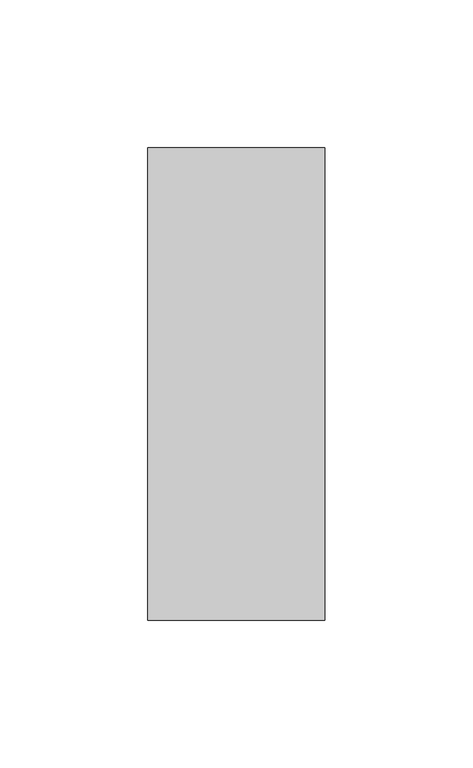
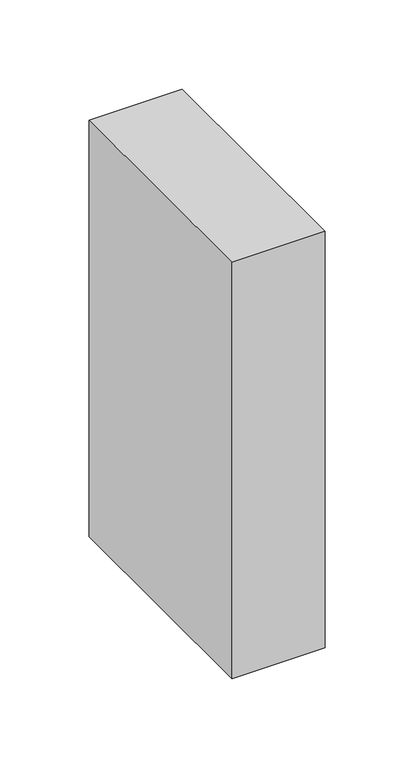
"""IFC4 building model written with IfcOpenShell, lengths in millimetres: column geometry, Madeira de lei-Coluna : Pontalete 6X16cm."""

import ifcopenshell
import ifcopenshell.guid

model = None  # the IFC model being written
_history = None  # IfcOwnerHistory: only IFC2X3 demands one
_inside = {}  # id of a spatial element -> (the spatial element, [elements in it])
_under = {}  # id of a project, library or spatial element -> (it, [spatial elements below it])
_declared = {}  # id of a project -> (the project, [libraries it declares])
_typed = {}  # id of a type object -> (the type object, [elements of that type])
_made_of = {}  # id of a material, layer set ... -> (it, [elements and type objects made of it])


def new_model(schema):
    """Start an empty IFC model of exactly this schema.

    Asked for "IFC4X3", IfcOpenShell would pick the latest addendum, in which some entities
    have other attributes; the version numbers below select the first issue.
    IFC2X3 requires an IfcOwnerHistory on every rooted entity: one is made here for all.
    """
    global model, _history
    if schema == "IFC4X3":
        model = ifcopenshell.file(schema_version=(4, 3, 0, 0))
    else:
        model = ifcopenshell.file(schema=schema)
    _inside.clear()
    _under.clear()
    _declared.clear()
    _typed.clear()
    _made_of.clear()
    _history = None
    if model.schema == "IFC2X3":
        org = make("IfcOrganization", Name="unknown")
        user = make(
            "IfcPersonAndOrganization",
            ThePerson=make("IfcPerson", FamilyName="unknown"),
            TheOrganization=org,
        )
        app = make(
            "IfcApplication",
            ApplicationDeveloper=org,
            Version="unknown",
            ApplicationFullName="unknown",
            ApplicationIdentifier="unknown",
        )
        _history = make(
            "IfcOwnerHistory",
            OwningUser=user,
            OwningApplication=app,
            ChangeAction="ADDED",
            CreationDate=0,
        )
    return model


def make(cls, **values):
    """One entity of the class cls with the attributes given. An attribute that is None is left unset."""
    return model.create_entity(
        cls, **{name: value for name, value in values.items() if value is not None}
    )


def rooted(cls, **values):
    """An entity with a GlobalId (a new one), such as an element, a storey or a relation."""
    return make(cls, GlobalId=ifcopenshell.guid.new(), OwnerHistory=_history, **values)


def si_unit(unit_type, name, prefix=None):
    """IfcSIUnit, for example si_unit("LENGTHUNIT", "METRE", prefix="MILLI")."""
    return make("IfcSIUnit", UnitType=unit_type, Prefix=prefix, Name=name)


def assignment(units):
    """IfcUnitAssignment: the units of a project."""
    return None if units is None else make("IfcUnitAssignment", Units=units)


def point(xyz):
    """IfcCartesianPoint."""
    return None if xyz is None else make("IfcCartesianPoint", Coordinates=xyz)


def direction(xyz):
    """IfcDirection."""
    return None if xyz is None else make("IfcDirection", DirectionRatios=xyz)


def frame(location, z_axis=None, x_axis=None):
    """IfcAxis2Placement3D, a coordinate frame: its origin and axes. An axis left out is left unset."""
    return make(
        "IfcAxis2Placement3D",
        Location=point(location),
        Axis=direction(z_axis),
        RefDirection=direction(x_axis),
    )


def origin():
    """The frame at (0, 0, 0) with its axes left unset."""
    return frame((0.0, 0.0, 0.0))


def place(relative_to, where):
    """IfcLocalPlacement: puts the frame where relative to a parent placement (None: the world)."""
    return make(
        "IfcLocalPlacement", PlacementRelTo=relative_to, RelativePlacement=where
    )


def context(
    kind, dimensions, precision=None, world=None, true_north=None, identifier=None
):
    """IfcGeometricRepresentationContext, for example the 3D "Model" context."""
    return make(
        "IfcGeometricRepresentationContext",
        ContextIdentifier=identifier,
        ContextType=kind,
        CoordinateSpaceDimension=dimensions,
        Precision=precision,
        WorldCoordinateSystem=world,
        TrueNorth=true_north,
    )


def project(units=None, contexts=None):
    """IfcProject with its units and contexts."""
    return rooted(
        "IfcProject",
        Name="project",
        RepresentationContexts=contexts,
        UnitsInContext=assignment(units),
    )


def spatial(cls, under=None, at=None, **own):
    """A site, building, storey or space (cls), placed at a placement, below another one or the project."""
    s = rooted(cls, ObjectPlacement=at, **own)
    if under is not None:
        _under.setdefault(under.id(), (under, []))[1].append(s)
    return s


def polyline(points):
    """IfcPolyline through the points."""
    return make("IfcPolyline", Points=[point(p) for p in points])


def outline(outer, holes=None, kind="AREA"):
    """IfcArbitraryClosedProfileDef: a profile drawn as a closed curve; with holes, ...WithVoids."""
    if holes is None:
        return make("IfcArbitraryClosedProfileDef", ProfileType=kind, OuterCurve=outer)
    return make(
        "IfcArbitraryProfileDefWithVoids",
        ProfileType=kind,
        OuterCurve=outer,
        InnerCurves=holes,
    )


def extrude(swept, where, along, depth):
    """IfcExtrudedAreaSolid: the profile swept, set in the frame where, extruded along a direction by depth."""
    return make(
        "IfcExtrudedAreaSolid",
        SweptArea=swept,
        Position=where,
        ExtrudedDirection=direction(along),
        Depth=depth,
    )


def shape(context_of_items, identifier, shape_type, items):
    """IfcShapeRepresentation: the items that make up one representation, for example the "Body"."""
    return make(
        "IfcShapeRepresentation",
        ContextOfItems=context_of_items,
        RepresentationIdentifier=identifier,
        RepresentationType=shape_type,
        Items=items,
    )


def source(mapping_origin, context_of_items, identifier, shape_type, items):
    """IfcRepresentationMap: a shape defined once, which mapped items show again and again."""
    return make(
        "IfcRepresentationMap",
        MappingOrigin=mapping_origin,
        MappedRepresentation=shape(context_of_items, identifier, shape_type, items),
    )


def transform(
    local_origin,
    x_axis=None,
    y_axis=None,
    z_axis=None,
    scale=None,
    scale2=None,
    scale3=None,
    uniform=True,
):
    """IfcCartesianTransformationOperator3D, or its non-uniform kind. x_axis, y_axis, z_axis: its Axis1, 2, 3."""
    if uniform:
        return make(
            "IfcCartesianTransformationOperator3D",
            Axis1=direction(x_axis),
            Axis2=direction(y_axis),
            LocalOrigin=point(local_origin),
            Scale=scale,
            Axis3=direction(z_axis),
        )
    return make(
        "IfcCartesianTransformationOperator3DnonUniform",
        Axis1=direction(x_axis),
        Axis2=direction(y_axis),
        LocalOrigin=point(local_origin),
        Scale=scale,
        Axis3=direction(z_axis),
        Scale2=scale2,
        Scale3=scale3,
    )


def mapped(mapping_source, mapping_target):
    """IfcMappedItem: shows the shape of a source again, moved by a transform."""
    return make(
        "IfcMappedItem", MappingSource=mapping_source, MappingTarget=mapping_target
    )


def made_of(thing, what):
    """Note that an element or type object is made of a material, layer set ...; save() writes the relation."""
    if what is not None:
        _made_of.setdefault(what.id(), (what, []))[1].append(thing)
    return thing


def element(
    cls,
    number,
    at=None,
    inside=None,
    cuts=None,
    type_object=None,
    material=None,
    context=None,
    identifier="Body",
    shape_type=None,
    held_by="IfcProductDefinitionShape",
    body=None,
    shapes=None,
    **own,
):
    """One element of the class cls, such as IfcWall. Its Tag is "e" and its number.

    at: its placement. inside: the storey or other place that contains it. cuts: it is an
    opening in that element (IfcRelVoidsElement). A single representation is given by context,
    identifier, shape_type and body (its items); several are given by shapes. held_by: the class
    of the entity that holds the representations. save() writes the other relations.
    """
    e = rooted(cls, Tag="e%d" % number, ObjectPlacement=at, **own)
    if body is not None:
        shapes = [shape(context, identifier, shape_type, body)]
    if shapes is not None:
        e.Representation = make(held_by, Representations=shapes)
    if inside is not None:
        _inside.setdefault(inside.id(), (inside, []))[1].append(e)
    if cuts is not None:
        rooted(
            "IfcRelVoidsElement", RelatingBuildingElement=cuts, RelatedOpeningElement=e
        )
    if type_object is not None:
        _typed.setdefault(type_object.id(), (type_object, []))[1].append(e)
    return made_of(e, material)


def aggregate(whole, parts):
    """IfcRelAggregates: a whole, such as a stair, and the parts it consists of."""
    return rooted("IfcRelAggregates", RelatingObject=whole, RelatedObjects=parts)


def save(model, path):
    """Write the relations noted so far, then the file.

    IfcRelAggregates (storeys below a building ...), IfcRelContainedInSpatialStructure (elements
    in a storey), IfcRelDefinesByType, IfcRelAssociatesMaterial and IfcRelDeclares: one each for
    every whole, place, type object, material and project.
    """
    for whole, parts in _under.values():
        aggregate(whole, parts)
    for where, things in _inside.values():
        rooted(
            "IfcRelContainedInSpatialStructure",
            RelatedElements=things,
            RelatingStructure=where,
        )
    for kind, things in _typed.values():
        rooted("IfcRelDefinesByType", RelatedObjects=things, RelatingType=kind)
    for what, things in _made_of.values():
        rooted("IfcRelAssociatesMaterial", RelatedObjects=things, RelatingMaterial=what)
    for by, libraries in _declared.values():
        rooted("IfcRelDeclares", RelatingContext=by, RelatedDefinitions=libraries)
    model.write(path)


def column_1adb463a(model_context):
    return source(origin(), model_context, "Body", "SweptSolid", [
        extrude(outline(polyline([(30.0, 80.0), (30.0, -80.0), (-30.0, -80.0), (-30.0, 80.0), (30.0, 80.0)])), frame((0.0, 0.0, 6710.0), z_axis=(0.0, 0.0, 1.0), x_axis=(1.0, 0.0, 0.0)), (0.0, 0.0, 1.0), 284.6),
    ])


if __name__ == "__main__":
    model = new_model("IFC4")
    model_context = context("Model", 3, world=origin())
    ifc_project = project(units=[si_unit("LENGTHUNIT", "METRE", prefix="MILLI")], contexts=[model_context])
    site = spatial("IfcSite", under=ifc_project)
    building = spatial("IfcBuilding", under=site)
    placement = place(None, origin())
    column_shape = column_1adb463a(model_context)
    element("IfcColumn", 1, ObjectType="Madeira de lei-Coluna : Pontalete 6X16cm", at=placement, inside=building, context=model_context, shape_type="MappedRepresentation", body=[
        mapped(column_shape, transform((0.0, 0.0, 0.0), x_axis=(1.0, 0.0, 0.0), y_axis=(0.0, 1.0, 0.0), z_axis=(0.0, 0.0, 1.0))),
    ])
    save(model, "model.ifc")

# Revit data of these elements
# Project information
#   Design Option = "Main Model"
#   Project Status = "Status do projeto"
#   Client Name = "JOÃO MATIAS SOARES"
#   Project Address = "RUA SÉRGIO DIAS, LOTE 30, QUADRA G, MONTE MINEIRO/MG"
#   Project Name = "CONSTRUÇÃO RESIDENCIA UNIFAMILIAR"
#   Project Number = "034/2017"
#   Zona = "ZER - 01"
#   CA Mín = "0.2"
#   CA Básico = "1"
#   CA Máx = "2"
#   TO Máx = "50"
#   Gabarito Máx = "10"
#   TP Mín = "15"
#   Área Total do Terreno = "620.00 m²"
#   Multifamiliar - Vagas Veículos/Pavto = "0"
#   Multifamiliar - Vagas Bicicletas/Pavto = "0"
#   Multifamiliar - % Vagas PNMR = "0"
#   Multifamiliar - % Vagas Motos = "0"
#   Outros - Área p/ 1 Veículo = "0.00 m²"
#   Outros - Área p/ 1 Bicicleta = "0.00 m²"
#   Outros - Área p/ 1 Utilitário = "0.00 m²"
#   Outros - % Vagas PNMR = "0"
#   Outros - % Vagas Motos = "0"
# Type "Madeira de lei-Coluna : Pontalete 6X16cm"
#   A = 0.01952 m²
#   b = 0.06 m
#   d = 0.16 m
#   Structural Material [instance default] = none
#   Assembly Code = ""
# Element 1 (IfcColumn, "Madeira de lei-Coluna : Pontalete 6X16cm")
#   Structural Material = .MADEIRAMENTO
#   Materials on its faces: ".MADEIRAMENTO"
# Materials
#   ".MADEIRAMENTO": class ".CC_MADEIRAS", colour RGB 212 179 113, transparency 0, Cost = 0
